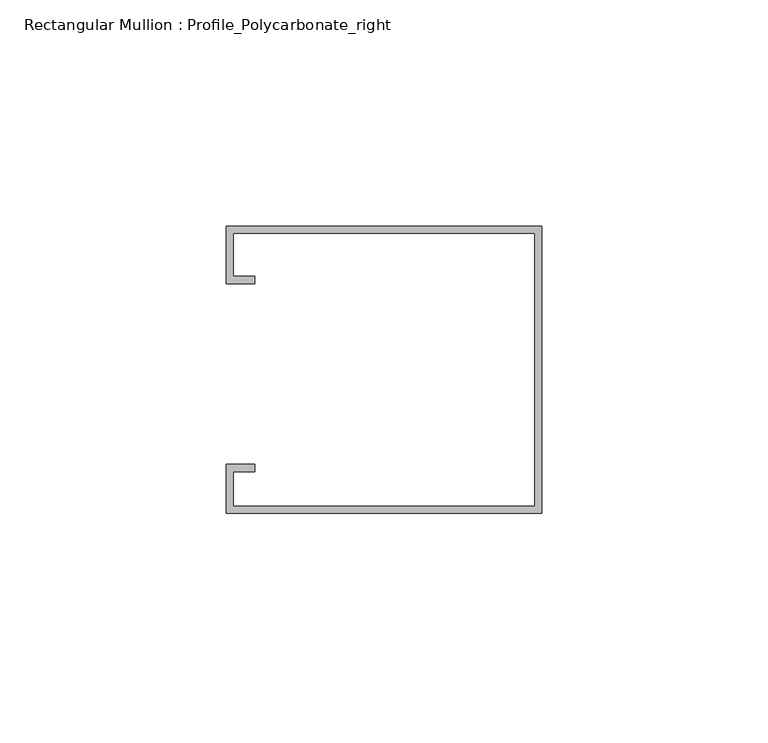
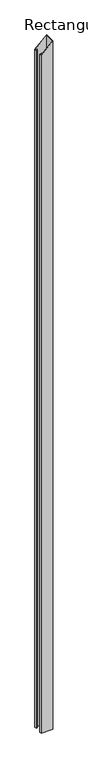
"""IFC4 building model written with IfcOpenShell, lengths in millimetres: member geometry, Rectangular Mullion : Profile_Polycarbonate_right."""

from ifc_helpers import new_model, si_unit, origin, place, context, project, spatial, faceted_brep, source, transform, mapped, element, save


def rectangular_mullion_profile_polycarbonate_right_2d9b79c2(model_context):
    return source(origin(), model_context, "Body", "Brep", [
        faceted_brep([(0.0, 32.7, -4369.9243931), (0.0, -30.8, -4369.9243931), (-69.85, -30.8, -4369.9243931), (-69.85, -20.0, -4369.9243931), (-63.5, -20.0, -4369.9243931), (-63.5, -21.5875, -4369.9243931), (-68.2625, -21.5875, -4369.9243931), (-68.2625, -29.2125, -4369.9243931), (-1.5875, -29.2125, -4369.9243931), (-1.5875, 31.1125, -4369.9243931), (-68.2625, 31.1125, -4369.9243931), (-68.2625, 21.5875, -4369.9243931), (-63.5, 21.5875, -4369.9243931), (-63.5, 20.0, -4369.9243931), (-69.85, 20.0, -4369.9243931), (-69.85, 32.7, -4369.9243931), (-69.85, 32.7, -67.0001907), (0.0, 32.7, 0.0), (-69.85, 20.0, -67.0001907), (-63.5, 20.0, -60.9092643), (-63.5, 21.5875, -60.9092643), (-68.2625, 21.5875, -65.4774591), (-68.2625, 31.1125, -65.4774591), (-1.5875, 31.1125, -1.5227316), (-1.5875, -29.2125, -1.5227316), (-68.2625, -29.2125, -65.4774591), (-68.2625, -21.5875, -65.4774591), (-63.5, -21.5875, -60.9092643), (-63.5, -20.0, -60.9092643), (-69.85, -20.0, -67.0001907), (-69.85, -30.8, -67.0001907), (0.0, -30.8, 0.0)], [[[0, 1, 2, 3, 4, 5, 6, 7, 8, 9, 10, 11, 12, 13, 14, 15]], [[16, 17, 0, 15]], [[18, 16, 15, 14]], [[19, 18, 14, 13]], [[20, 19, 13, 12]], [[21, 20, 12, 11]], [[22, 21, 11, 10]], [[23, 22, 10, 9]], [[24, 23, 9, 8]], [[25, 24, 8, 7]], [[26, 25, 7, 6]], [[27, 26, 6, 5]], [[28, 27, 5, 4]], [[29, 28, 4, 3]], [[30, 29, 3, 2]], [[31, 30, 2, 1]], [[17, 31, 1, 0]], [[17, 16, 18, 19, 20, 21, 22, 23, 24, 25, 26, 27, 28, 29, 30, 31]]]),
    ])


if __name__ == "__main__":
    model = new_model("IFC4")
    model_context = context("Model", 3, world=origin())
    ifc_project = project(units=[si_unit("LENGTHUNIT", "METRE", prefix="MILLI")], contexts=[model_context])
    site = spatial("IfcSite", under=ifc_project)
    building = spatial("IfcBuilding", under=site)
    placement = place(None, origin())
    rectangular_mullion_profile_polycarbonate_right_shape = rectangular_mullion_profile_polycarbonate_right_2d9b79c2(model_context)
    element("IfcMember", 1, ObjectType="Rectangular Mullion : Profile_Polycarbonate_right", at=placement, inside=building, context=model_context, shape_type="MappedRepresentation", body=[
        mapped(rectangular_mullion_profile_polycarbonate_right_shape, transform((0.0, 0.0, 0.0), x_axis=(1.0, 0.0, 0.0), y_axis=(0.0, 1.0, 0.0), z_axis=(0.0, 0.0, 1.0))),
    ])
    save(model, "model.ifc")

# Revit data of these elements
# Type "Rectangular Mullion : Profile_Polycarbonate_right"
#   built-in parameter 1007322 = 0.208333 (stored number, unit not read)
#   built-in parameter 1007321 = 0 (stored number, unit not read)
#   built-in parameter 1007320 = 0.00520833 (stored number, unit not read)
